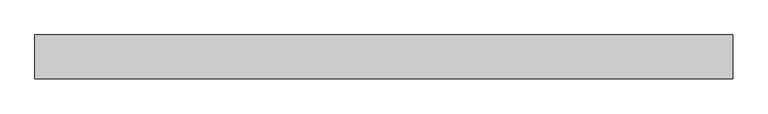
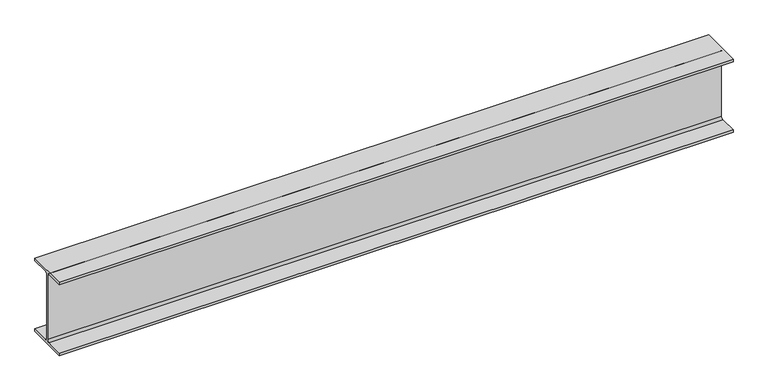
"""IFC4 building model written with IfcOpenShell, lengths in millimetres: beam geometry, Old_Steel Beam_H-KSD3502 : H_SB_ASB_H-200×200x8x12."""

from ifc_helpers import new_model, si_unit, point, frame, frame_2d, origin, place, context, project, spatial, polyline, circle_curve, trimmed, segment, composite_curve, outline, extrude, source, transform, mapped, element, save


def beam_5a985b38(model_context):
    return source(origin(), model_context, "Body", "SweptSolid", [
        extrude(outline(composite_curve([segment(polyline([(82.5, -141.5), (82.5, -151.7), (-82.5, -151.7), (-82.5, -141.5), (-11.9, -141.5)]), True, "CONTINUOUS"), segment(trimmed(circle_curve(frame_2d((-11.9, -132.6)), 8.9), [point((-11.9, -141.5))], [point((-3.0, -132.6))], True, "CARTESIAN"), True, "CONTINUOUS"), segment(polyline([(-3.0, -132.6), (-3.0, 132.6)]), True, "CONTINUOUS"), segment(trimmed(circle_curve(frame_2d((-11.9, 132.6)), 8.9), [point((-3.0, 132.6))], [point((-11.9, 141.5))], True, "CARTESIAN"), True, "CONTINUOUS"), segment(polyline([(-11.9, 141.5), (-82.5, 141.5), (-82.5, 151.7), (82.5, 151.7), (82.5, 141.5), (11.9, 141.5)]), True, "CONTINUOUS"), segment(trimmed(circle_curve(frame_2d((11.9, 132.6)), 8.9), [point((11.9, 141.5))], [point((3.0, 132.6))], True, "CARTESIAN"), True, "CONTINUOUS"), segment(polyline([(3.0, 132.6), (3.0, -132.6)]), True, "CONTINUOUS"), segment(trimmed(circle_curve(frame_2d((11.9, -132.6)), 8.9), [point((3.0, -132.6))], [point((11.9, -141.5))], True, "CARTESIAN"), True, "CONTINUOUS"), segment(polyline([(11.9, -141.5), (82.5, -141.5)]), True, "CONTINUOUS")], self_intersect=False)), frame((-1301.2819018, 0.0, 0.0), z_axis=(1.0, 0.0, 0.0), x_axis=(0.0, 1.0, 0.0)), (0.0, 0.0, 1.0), 2636.1330811),
    ])


if __name__ == "__main__":
    model = new_model("IFC4")
    model_context = context("Model", 3, world=origin())
    ifc_project = project(units=[si_unit("LENGTHUNIT", "METRE", prefix="MILLI")], contexts=[model_context])
    site = spatial("IfcSite", under=ifc_project)
    building = spatial("IfcBuilding", under=site)
    placement = place(None, origin())
    beam_shape = beam_5a985b38(model_context)
    element("IfcBeam", 1, ObjectType="Old_Steel Beam_H-KSD3502 : H_SB_ASB_H-200×200x8x12", at=placement, inside=building, context=model_context, shape_type="MappedRepresentation", body=[
        mapped(beam_shape, transform((0.0, 0.0, 0.0), x_axis=(1.0, 0.0, 0.0), y_axis=(0.0, 1.0, 0.0), z_axis=(0.0, 0.0, 1.0))),
    ])
    save(model, "model.ifc")

# Revit data of these elements
# Type "Old_Steel Beam_H-KSD3502 : H_SB_ASB_H-200×200x8x12"
#   Width = 20.0 cm
#   Web Thickness = 0.8 cm
#   Web Fillet = 1.3 cm
#   Warping Constant = 141376.0 cm⁶
#   Torsional Moment of Inertia = 26.2485 cm⁴
#   Torsional Modulus = 1.0 cm³
#   Section Area = 63.53 cm²
#   Plastic Modulus weak axis = 244.0 cm³
#   Plastic Modulus strong axis = 525.0 cm³
#   Perimeter = 1.16 m²/m
#   Nominal Weight = 49.90 kgf/m
#   Moment of Inertia weak axis = 1600.00 cm⁴
#   Moment of Inertia strong axis = 4720.00 cm⁴
#   Height = 20.0 cm
#   Flange Thickness = 1.2 cm
#   Elastic Modulus weak axis = 160.0 cm³
#   Elastic Modulus strong axis = 472.0 cm³
#   Centroid Vertical = 10.0 cm
#   Centroid Horizontal = 10.0 cm
#   Length [instance default] = 1.5240 m
#   Structural Material [instance default] = Steel, 45-345
#   Assembly Code = ""
# Element 1 (IfcBeam, "Old_Steel Beam_H-KSD3502 : H_SB_ASB_H-200×200x8x12")
#   Structural Material = none
# Materials
#   "Steel, 45-345": class "Metal", colour RGB 189 187 185, transparency 0, Description = "Steel 345 MPa", Cost = 0
